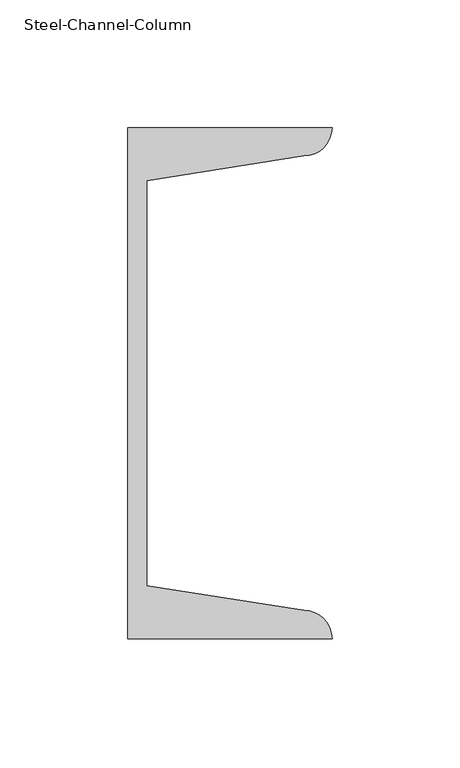
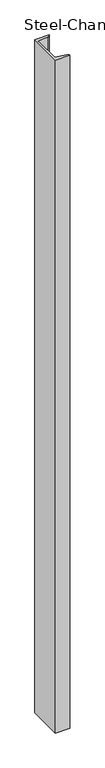
"""IFC4 building model written with IfcOpenShell, lengths in millimetres: column geometry, Steel-Channel-Column : CL126_C-200×80x7.5x11."""

import ifcopenshell
import ifcopenshell.guid

model = None  # the IFC model being written
_history = None  # IfcOwnerHistory: only IFC2X3 demands one
_inside = {}  # id of a spatial element -> (the spatial element, [elements in it])
_under = {}  # id of a project, library or spatial element -> (it, [spatial elements below it])
_declared = {}  # id of a project -> (the project, [libraries it declares])
_typed = {}  # id of a type object -> (the type object, [elements of that type])
_made_of = {}  # id of a material, layer set ... -> (it, [elements and type objects made of it])


def new_model(schema):
    """Start an empty IFC model of exactly this schema.

    Asked for "IFC4X3", IfcOpenShell would pick the latest addendum, in which some entities
    have other attributes; the version numbers below select the first issue.
    IFC2X3 requires an IfcOwnerHistory on every rooted entity: one is made here for all.
    """
    global model, _history
    if schema == "IFC4X3":
        model = ifcopenshell.file(schema_version=(4, 3, 0, 0))
    else:
        model = ifcopenshell.file(schema=schema)
    _inside.clear()
    _under.clear()
    _declared.clear()
    _typed.clear()
    _made_of.clear()
    _history = None
    if model.schema == "IFC2X3":
        org = make("IfcOrganization", Name="unknown")
        user = make(
            "IfcPersonAndOrganization",
            ThePerson=make("IfcPerson", FamilyName="unknown"),
            TheOrganization=org,
        )
        app = make(
            "IfcApplication",
            ApplicationDeveloper=org,
            Version="unknown",
            ApplicationFullName="unknown",
            ApplicationIdentifier="unknown",
        )
        _history = make(
            "IfcOwnerHistory",
            OwningUser=user,
            OwningApplication=app,
            ChangeAction="ADDED",
            CreationDate=0,
        )
    return model


def make(cls, **values):
    """One entity of the class cls with the attributes given. An attribute that is None is left unset."""
    return model.create_entity(
        cls, **{name: value for name, value in values.items() if value is not None}
    )


def rooted(cls, **values):
    """An entity with a GlobalId (a new one), such as an element, a storey or a relation."""
    return make(cls, GlobalId=ifcopenshell.guid.new(), OwnerHistory=_history, **values)


def si_unit(unit_type, name, prefix=None):
    """IfcSIUnit, for example si_unit("LENGTHUNIT", "METRE", prefix="MILLI")."""
    return make("IfcSIUnit", UnitType=unit_type, Prefix=prefix, Name=name)


def assignment(units):
    """IfcUnitAssignment: the units of a project."""
    return None if units is None else make("IfcUnitAssignment", Units=units)


def point(xyz):
    """IfcCartesianPoint."""
    return None if xyz is None else make("IfcCartesianPoint", Coordinates=xyz)


def direction(xyz):
    """IfcDirection."""
    return None if xyz is None else make("IfcDirection", DirectionRatios=xyz)


def frame(location, z_axis=None, x_axis=None):
    """IfcAxis2Placement3D, a coordinate frame: its origin and axes. An axis left out is left unset."""
    return make(
        "IfcAxis2Placement3D",
        Location=point(location),
        Axis=direction(z_axis),
        RefDirection=direction(x_axis),
    )


def frame_2d(location, x_axis=None):
    """IfcAxis2Placement2D, a coordinate frame in the plane: its origin and x axis."""
    return make(
        "IfcAxis2Placement2D", Location=point(location), RefDirection=direction(x_axis)
    )


def origin():
    """The frame at (0, 0, 0) with its axes left unset."""
    return frame((0.0, 0.0, 0.0))


def origin_with_axes():
    """The frame at (0, 0, 0) with the z axis (0, 0, 1) and the x axis (1, 0, 0) written out."""
    return frame((0.0, 0.0, 0.0), z_axis=(0.0, 0.0, 1.0), x_axis=(1.0, 0.0, 0.0))


def place(relative_to, where):
    """IfcLocalPlacement: puts the frame where relative to a parent placement (None: the world)."""
    return make(
        "IfcLocalPlacement", PlacementRelTo=relative_to, RelativePlacement=where
    )


def context(
    kind, dimensions, precision=None, world=None, true_north=None, identifier=None
):
    """IfcGeometricRepresentationContext, for example the 3D "Model" context."""
    return make(
        "IfcGeometricRepresentationContext",
        ContextIdentifier=identifier,
        ContextType=kind,
        CoordinateSpaceDimension=dimensions,
        Precision=precision,
        WorldCoordinateSystem=world,
        TrueNorth=true_north,
    )


def project(units=None, contexts=None):
    """IfcProject with its units and contexts."""
    return rooted(
        "IfcProject",
        Name="project",
        RepresentationContexts=contexts,
        UnitsInContext=assignment(units),
    )


def spatial(cls, under=None, at=None, **own):
    """A site, building, storey or space (cls), placed at a placement, below another one or the project."""
    s = rooted(cls, ObjectPlacement=at, **own)
    if under is not None:
        _under.setdefault(under.id(), (under, []))[1].append(s)
    return s


def polyline(points):
    """IfcPolyline through the points."""
    return make("IfcPolyline", Points=[point(p) for p in points])


def circle_curve(where, radius):
    """IfcCircle in the frame where."""
    return make("IfcCircle", Position=where, Radius=radius)


def trimmed(basis, trim1, trim2, sense, master):
    """IfcTrimmedCurve: the piece of a basis curve between two trims."""
    return make(
        "IfcTrimmedCurve",
        BasisCurve=basis,
        Trim1=trim1,
        Trim2=trim2,
        SenseAgreement=sense,
        MasterRepresentation=master,
    )


def segment(curve, same_sense, transition):
    """IfcCompositeCurveSegment."""
    return make(
        "IfcCompositeCurveSegment",
        Transition=transition,
        SameSense=same_sense,
        ParentCurve=curve,
    )


def composite_curve(segments, self_intersect=None):
    """IfcCompositeCurve: segments joined end to end."""
    return make("IfcCompositeCurve", Segments=segments, SelfIntersect=self_intersect)


def outline(outer, holes=None, kind="AREA"):
    """IfcArbitraryClosedProfileDef: a profile drawn as a closed curve; with holes, ...WithVoids."""
    if holes is None:
        return make("IfcArbitraryClosedProfileDef", ProfileType=kind, OuterCurve=outer)
    return make(
        "IfcArbitraryProfileDefWithVoids",
        ProfileType=kind,
        OuterCurve=outer,
        InnerCurves=holes,
    )


def extrude(swept, where, along, depth):
    """IfcExtrudedAreaSolid: the profile swept, set in the frame where, extruded along a direction by depth."""
    return make(
        "IfcExtrudedAreaSolid",
        SweptArea=swept,
        Position=where,
        ExtrudedDirection=direction(along),
        Depth=depth,
    )


def shape(context_of_items, identifier, shape_type, items):
    """IfcShapeRepresentation: the items that make up one representation, for example the "Body"."""
    return make(
        "IfcShapeRepresentation",
        ContextOfItems=context_of_items,
        RepresentationIdentifier=identifier,
        RepresentationType=shape_type,
        Items=items,
    )


def source(mapping_origin, context_of_items, identifier, shape_type, items):
    """IfcRepresentationMap: a shape defined once, which mapped items show again and again."""
    return make(
        "IfcRepresentationMap",
        MappingOrigin=mapping_origin,
        MappedRepresentation=shape(context_of_items, identifier, shape_type, items),
    )


def transform(
    local_origin,
    x_axis=None,
    y_axis=None,
    z_axis=None,
    scale=None,
    scale2=None,
    scale3=None,
    uniform=True,
):
    """IfcCartesianTransformationOperator3D, or its non-uniform kind. x_axis, y_axis, z_axis: its Axis1, 2, 3."""
    if uniform:
        return make(
            "IfcCartesianTransformationOperator3D",
            Axis1=direction(x_axis),
            Axis2=direction(y_axis),
            LocalOrigin=point(local_origin),
            Scale=scale,
            Axis3=direction(z_axis),
        )
    return make(
        "IfcCartesianTransformationOperator3DnonUniform",
        Axis1=direction(x_axis),
        Axis2=direction(y_axis),
        LocalOrigin=point(local_origin),
        Scale=scale,
        Axis3=direction(z_axis),
        Scale2=scale2,
        Scale3=scale3,
    )


def mapped(mapping_source, mapping_target):
    """IfcMappedItem: shows the shape of a source again, moved by a transform."""
    return make(
        "IfcMappedItem", MappingSource=mapping_source, MappingTarget=mapping_target
    )


def made_of(thing, what):
    """Note that an element or type object is made of a material, layer set ...; save() writes the relation."""
    if what is not None:
        _made_of.setdefault(what.id(), (what, []))[1].append(thing)
    return thing


def element(
    cls,
    number,
    at=None,
    inside=None,
    cuts=None,
    type_object=None,
    material=None,
    context=None,
    identifier="Body",
    shape_type=None,
    held_by="IfcProductDefinitionShape",
    body=None,
    shapes=None,
    **own,
):
    """One element of the class cls, such as IfcWall. Its Tag is "e" and its number.

    at: its placement. inside: the storey or other place that contains it. cuts: it is an
    opening in that element (IfcRelVoidsElement). A single representation is given by context,
    identifier, shape_type and body (its items); several are given by shapes. held_by: the class
    of the entity that holds the representations. save() writes the other relations.
    """
    e = rooted(cls, Tag="e%d" % number, ObjectPlacement=at, **own)
    if body is not None:
        shapes = [shape(context, identifier, shape_type, body)]
    if shapes is not None:
        e.Representation = make(held_by, Representations=shapes)
    if inside is not None:
        _inside.setdefault(inside.id(), (inside, []))[1].append(e)
    if cuts is not None:
        rooted(
            "IfcRelVoidsElement", RelatingBuildingElement=cuts, RelatedOpeningElement=e
        )
    if type_object is not None:
        _typed.setdefault(type_object.id(), (type_object, []))[1].append(e)
    return made_of(e, material)


def aggregate(whole, parts):
    """IfcRelAggregates: a whole, such as a stair, and the parts it consists of."""
    return rooted("IfcRelAggregates", RelatingObject=whole, RelatedObjects=parts)


def save(model, path):
    """Write the relations noted so far, then the file.

    IfcRelAggregates (storeys below a building ...), IfcRelContainedInSpatialStructure (elements
    in a storey), IfcRelDefinesByType, IfcRelAssociatesMaterial and IfcRelDeclares: one each for
    every whole, place, type object, material and project.
    """
    for whole, parts in _under.values():
        aggregate(whole, parts)
    for where, things in _inside.values():
        rooted(
            "IfcRelContainedInSpatialStructure",
            RelatedElements=things,
            RelatingStructure=where,
        )
    for kind, things in _typed.values():
        rooted("IfcRelDefinesByType", RelatedObjects=things, RelatingType=kind)
    for what, things in _made_of.values():
        rooted("IfcRelAssociatesMaterial", RelatedObjects=things, RelatingMaterial=what)
    for by, libraries in _declared.values():
        rooted("IfcRelDeclares", RelatingContext=by, RelatedDefinitions=libraries)
    model.write(path)


def steel_channel_column_12e21b6e(model_context):
    return source(origin(), model_context, "Body", "SweptSolid", [
        extrude(outline(composite_curve([segment(polyline([(-22.1, 100.0), (57.9, 100.0)]), True, "CONTINUOUS"), segment(trimmed(circle_curve(frame_2d((46.9, 100.0)), 11.0), [point((57.9, 100.0))], [point((46.9, 89.0))], False, "CARTESIAN"), True, "CONTINUOUS"), segment(polyline([(46.9, 89.0), (-14.6, 79.2593569), (-14.6, -79.2593569), (46.9, -89.0)]), True, "CONTINUOUS"), segment(trimmed(circle_curve(frame_2d((46.9, -100.0)), 11.0), [point((46.9, -89.0))], [point((57.9, -100.0))], False, "CARTESIAN"), True, "CONTINUOUS"), segment(polyline([(57.9, -100.0), (-22.1, -100.0), (-22.1, 100.0)]), True, "CONTINUOUS")], self_intersect=False)), origin_with_axes(), (0.0, 0.0, 1.0), 4000.0),
    ])


if __name__ == "__main__":
    model = new_model("IFC4")
    model_context = context("Model", 3, world=origin())
    ifc_project = project(units=[si_unit("LENGTHUNIT", "METRE", prefix="MILLI")], contexts=[model_context])
    site = spatial("IfcSite", under=ifc_project)
    building = spatial("IfcBuilding", under=site)
    placement = place(None, origin())
    steel_channel_column_shape = steel_channel_column_12e21b6e(model_context)
    element("IfcColumn", 1, ObjectType="Steel-Channel-Column : CL126_C-200×80x7.5x11", at=placement, inside=building, context=model_context, shape_type="MappedRepresentation", body=[
        mapped(steel_channel_column_shape, transform((0.0, 0.0, 0.0), x_axis=(1.0, 0.0, 0.0), y_axis=(0.0, 1.0, 0.0), z_axis=(0.0, 0.0, 1.0))),
    ])
    save(model, "model.ifc")

# Revit data of these elements
# Type "Steel-Channel-Column : CL126_C-200×80x7.5x11"
#   Assembly Code = "B10"
#   x = 22.1 mm
#   Section Area = 31.33 cm²
#   Mass per Unit Length = 24.60 kg/m
#   bf = 80 mm
#   d = 200 mm
#   tf = 11 mm
#   tw = 7.5 mm
#   hec_material4 [instance default] = none
#   hec_material3 [instance default] = none
#   hec_material2 [instance default] = none
#   hec_material1 [instance default] = none
#   Structural Material [instance default] = Steel, 45-345
# Element 1 (IfcColumn, "Steel-Channel-Column : CL126_C-200×80x7.5x11")
#   Materials on its faces: "Steel, 45-345"
# Materials
#   "Steel, 45-345": class "Metal", colour RGB 189 187 185, transparency 0, Description = "Steel 345 MPa", Cost = 0
